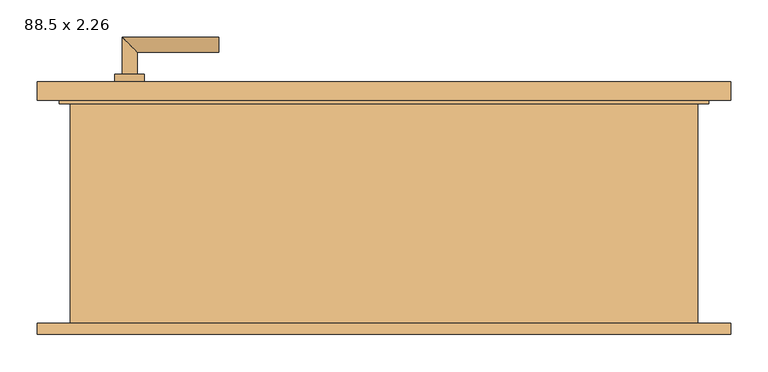
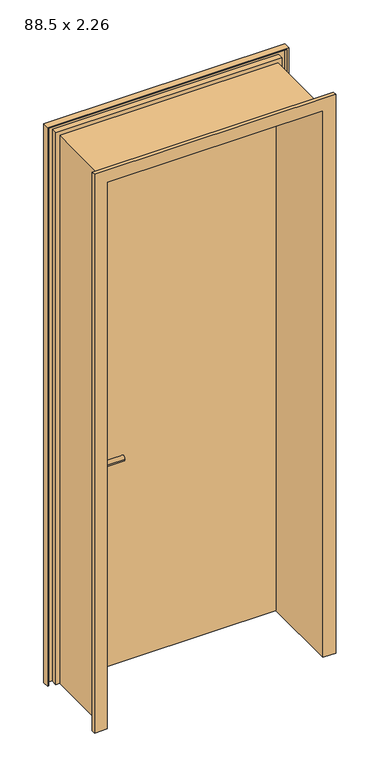
"""IFC4 building model written with IfcOpenShell, lengths in millimetres: door geometry, Drehflügel 1-flg - Stahlzarge : 88.5 x 2.26."""

from ifc_helpers import new_model, si_unit, point, frame, frame_2d, origin, origin_with_axes, place, context, project, spatial, polyline, circle_curve, ellipse_curve, trimmed, segment, composite_curve, outline, extrude, faceted_brep, source, transform, mapped, element, save
from ifc_brep_helpers import plane_surface, cylinder_surface, advanced_brep


def door_88_5_x_2_26_de88e540(model_context):
    return source(origin(), model_context, "Body", "SolidModel", [
        advanced_brep(
        [(-352.5, 139.4346141, 900.0), (-332.5, 139.4346141, 900.0), (-352.5, 69.4346141, 900.0), (-332.5, 89.4346141, 900.0), (-222.5, 69.4346141, 900.0), (-222.5, 89.4346141, 900.0)],
        [
            (0, 1, circle_curve(frame((-342.5, 139.4346141, 900.0), z_axis=(0.0, 1.0, 0.0), x_axis=(1.0, 0.0, 0.0)), 10.0)),
            (1, 0, circle_curve(frame((-342.5, 139.4346141, 900.0), z_axis=(0.0, 1.0, 0.0), x_axis=(1.0, 0.0, 0.0)), 10.0)),
            (0, 2),
            (2, 3, ellipse_curve(frame((-342.5, 79.4346141, 900.0), z_axis=(-0.7071067811865385, 0.7071067811865565, 0.0), x_axis=(0.7071067811865563, 0.7071067811865386, 0.0)), 14.1421356, 10.0)),
            (3, 1),
            (3, 2, ellipse_curve(frame((-342.5, 79.4346141, 900.0), z_axis=(-0.7071067811865385, 0.7071067811865565, 0.0), x_axis=(0.7071067811865563, 0.7071067811865386, 0.0)), 14.1421356, 10.0)),
            (4, 5, circle_curve(frame((-222.5, 79.4346141, 900.0), z_axis=(1.0, 0.0, 0.0), x_axis=(0.0, 1.0, 0.0)), 10.0)),
            (5, 4, circle_curve(frame((-222.5, 79.4346141, 900.0), z_axis=(1.0, 0.0, 0.0), x_axis=(0.0, 1.0, 0.0)), 10.0)),
            (2, 4),
            (5, 3),
        ],
        [
            plane_surface(frame((-342.5, 139.4346141, -387.7526403), z_axis=(0.0, 1.0, 0.0), x_axis=(0.0, 0.0, 1.0))),
            cylinder_surface(frame((-342.5, 139.4346141, 900.0), z_axis=(0.0, 1.0, 0.0), x_axis=(1.0, 0.0, 0.0)), 10.0),
            plane_surface(frame((-222.5, 79.4346141, -387.7526403), z_axis=(1.0, 0.0, 0.0), x_axis=(0.0, 0.0, 1.0))),
            cylinder_surface(frame((-342.5, 79.4346141, 900.0), z_axis=(-1.0, 0.0, 0.0), x_axis=(0.0, 1.0, 0.0)), 10.0),
        ],
        [
            (0, [[1, 2]]),
            (1, [[-1, 3, 4, 5]]),
            (1, [[-2, -5, 6, -3]]),
            (2, [[7, 8]]),
            (3, [[-4, 9, -8, 10]]),
            (3, [[-6, -10, -7, -9]]),
        ],
    ),
        advanced_brep(
        [(-332.5, 199.4346141, 900.0), (-352.5, 199.4346141, 900.0), (-332.5, 229.4346141, 900.0), (-352.5, 249.4346141, 900.0), (-222.5, 229.4346141, 900.0), (-222.5, 249.4346141, 900.0)],
        [
            (0, 1, circle_curve(frame((-342.5, 199.4346141, 900.0), z_axis=(0.0, -1.0, 0.0), x_axis=(-1.0, 0.0, 0.0)), 10.0)),
            (1, 0, circle_curve(frame((-342.5, 199.4346141, 900.0), z_axis=(0.0, -1.0, 0.0), x_axis=(-1.0, 0.0, 0.0)), 10.0)),
            (0, 2),
            (2, 3, ellipse_curve(frame((-342.5, 239.4346141, 900.0), z_axis=(-0.7071067811865475, -0.7071067811865475, 0.0), x_axis=(0.7071067811865474, -0.7071067811865476, 0.0)), 14.1421356, 10.0)),
            (3, 1),
            (3, 2, ellipse_curve(frame((-342.5, 239.4346141, 900.0), z_axis=(-0.7071067811865475, -0.7071067811865475, 0.0), x_axis=(0.7071067811865474, -0.7071067811865476, 0.0)), 14.1421356, 10.0)),
            (4, 5, circle_curve(frame((-222.5, 239.4346141, 900.0), z_axis=(1.0, 0.0, 0.0), x_axis=(0.0, 1.0, 0.0)), 10.0)),
            (5, 4, circle_curve(frame((-222.5, 239.4346141, 900.0), z_axis=(1.0, 0.0, 0.0), x_axis=(0.0, 1.0, 0.0)), 10.0)),
            (2, 4),
            (5, 3),
        ],
        [
            plane_surface(frame((-342.5, 199.4346141, -387.7526403), z_axis=(0.0, -1.0, 0.0), x_axis=(0.0, 0.0, 1.0))),
            cylinder_surface(frame((-342.5, 199.4346141, 900.0), z_axis=(0.0, -1.0, 0.0), x_axis=(-1.0, 0.0, 0.0)), 10.0),
            plane_surface(frame((-222.5, 239.4346141, -387.7526403), z_axis=(1.0, 0.0, 0.0), x_axis=(0.0, 0.0, 1.0))),
            cylinder_surface(frame((-342.5, 239.4346141, 900.0), z_axis=(-1.0, 0.0, 0.0), x_axis=(0.0, 1.0, 0.0)), 10.0),
        ],
        [
            (0, [[1, 2]]),
            (1, [[-1, 3, 4, 5]]),
            (1, [[-2, -5, 6, -3]]),
            (2, [[7, 8]]),
            (3, [[-4, 9, -8, 10]]),
            (3, [[-6, -10, -7, -9]]),
        ],
    ),
        extrude(outline(composite_curve([segment(trimmed(circle_curve(frame_2d((900.0, -342.5)), 20.0), [point((900.0, -362.5))], [point((900.0, -322.5))], False, "CARTESIAN"), True, "CONTINUOUS"), segment(trimmed(circle_curve(frame_2d((900.0, -342.5)), 20.0), [point((900.0, -322.5))], [point((900.0, -362.5))], False, "CARTESIAN"), True, "CONTINUOUS")], self_intersect=False)), frame((0.0, 129.4346141, 0.0), z_axis=(0.0, 1.0, 0.0), x_axis=(0.0, 0.0, 1.0)), (0.0, 0.0, 1.0), 10.0),
        extrude(outline(composite_curve([segment(trimmed(circle_curve(frame_2d((900.0, -342.5)), 20.0), [point((900.0, -362.5))], [point((900.0, -322.5))], False, "CARTESIAN"), True, "CONTINUOUS"), segment(trimmed(circle_curve(frame_2d((900.0, -342.5)), 20.0), [point((900.0, -322.5))], [point((900.0, -362.5))], False, "CARTESIAN"), True, "CONTINUOUS")], self_intersect=False)), frame((0.0, 189.4346141, 0.0), z_axis=(0.0, 1.0, 0.0), x_axis=(0.0, 0.0, 1.0)), (0.0, 0.0, 1.0), 10.0),
        extrude(outline(polyline([(432.5, 164.4346141), (-432.5, 164.4346141), (-432.5, 189.4346141), (432.5, 189.4346141), (432.5, 164.4346141)])), origin_with_axes(), (0.0, 0.0, 1.0), 2250.0),
        faceted_brep([(466.9603207, -150.5653859, 0.0), (417.5, -150.5653859, 0.0), (417.5, 164.4346141, 0.0), (432.5, 164.4346141, 0.0), (432.5, 189.4346141, 0.0), (466.9603207, 189.4346141, 0.0), (466.9603207, 164.4346141, 0.0), (461.9603207, 164.4346141, 0.0), (461.9603207, 184.4346141, 0.0), (437.5, 184.4346141, 0.0), (437.5, 159.4346141, 0.0), (422.5, 159.4346141, 0.0), (422.5, -145.5653859, 0.0), (461.9603207, -145.5653859, 0.0), (461.9603207, -135.5653859, 0.0), (466.9603207, -135.5653859, 0.0), (466.9603207, -150.5653859, 2284.4603207), (-466.9603207, -150.5653859, 2284.4603207), (-466.9603207, -150.5653859, 0.0), (-417.5, -150.5653859, 0.0), (-417.5, -150.5653859, 2235.0), (417.5, -150.5653859, 2235.0), (417.5, 164.4346141, 2235.0), (-417.5, 164.4346141, 2235.0), (-417.5, 164.4346141, 0.0), (-432.5, 164.4346141, 0.0), (-432.5, 164.4346141, 2250.0), (432.5, 164.4346141, 2250.0), (432.5, 189.4346141, 2250.0), (-432.5, 189.4346141, 2250.0), (-432.5, 189.4346141, 0.0), (-466.9603207, 189.4346141, 0.0), (-466.9603207, 189.4346141, 2284.4603207), (466.9603207, 189.4346141, 2284.4603207), (466.9603207, 164.4346141, 2284.4603207), (-466.9603207, 164.4346141, 2284.4603207), (-466.9603207, 164.4346141, 0.0), (-461.9603207, 164.4346141, 0.0), (-461.9603207, 164.4346141, 2279.4603207), (461.9603207, 164.4346141, 2279.4603207), (461.9603207, 184.4346141, 2279.4603207), (-461.9603207, 184.4346141, 2279.4603207), (-461.9603207, 184.4346141, 0.0), (-437.5, 184.4346141, 0.0), (-437.5, 184.4346141, 2255.0), (437.5, 184.4346141, 2255.0), (437.5, 159.4346141, 2255.0), (-437.5, 159.4346141, 2255.0), (-437.5, 159.4346141, 0.0), (-422.5, 159.4346141, 0.0), (-422.5, 159.4346141, 2240.0), (422.5, 159.4346141, 2240.0), (422.5, -145.5653859, 2240.0), (-422.5, -145.5653859, 2240.0), (-422.5, -145.5653859, 0.0), (-461.9603207, -145.5653859, 0.0), (-461.9603207, -145.5653859, 2279.4603207), (461.9603207, -145.5653859, 2279.4603207), (461.9603207, -135.5653859, 2279.4603207), (-461.9603207, -135.5653859, 2279.4603207), (-461.9603207, -135.5653859, 0.0), (-466.9603207, -135.5653859, 0.0), (-466.9603207, -135.5653859, 2284.4603207), (466.9603207, -135.5653859, 2284.4603207)], [[[0, 1, 2, 3, 4, 5, 6, 7, 8, 9, 10, 11, 12, 13, 14, 15]], [[1, 0, 16, 17, 18, 19, 20, 21]], [[2, 1, 21, 22]], [[3, 2, 22, 23, 24, 25, 26, 27]], [[4, 3, 27, 28]], [[5, 4, 28, 29, 30, 31, 32, 33]], [[6, 5, 33, 34]], [[7, 6, 34, 35, 36, 37, 38, 39]], [[8, 7, 39, 40]], [[9, 8, 40, 41, 42, 43, 44, 45]], [[10, 9, 45, 46]], [[11, 10, 46, 47, 48, 49, 50, 51]], [[12, 11, 51, 52]], [[13, 12, 52, 53, 54, 55, 56, 57]], [[14, 13, 57, 58]], [[15, 14, 58, 59, 60, 61, 62, 63]], [[0, 15, 63, 16]], [[17, 62, 61, 18]], [[18, 61, 60, 55, 54, 49, 48, 43, 42, 37, 36, 31, 30, 25, 24, 19]], [[23, 20, 19, 24]], [[29, 26, 25, 30]], [[35, 32, 31, 36]], [[41, 38, 37, 42]], [[47, 44, 43, 48]], [[53, 50, 49, 54]], [[59, 56, 55, 60]], [[22, 21, 20, 23]], [[28, 27, 26, 29]], [[34, 33, 32, 35]], [[40, 39, 38, 41]], [[46, 45, 44, 47]], [[52, 51, 50, 53]], [[58, 57, 56, 59]], [[16, 63, 62, 17]]]),
    ])


if __name__ == "__main__":
    model = new_model("IFC4")
    model_context = context("Model", 3, world=origin())
    ifc_project = project(units=[si_unit("LENGTHUNIT", "METRE", prefix="MILLI")], contexts=[model_context])
    site = spatial("IfcSite", under=ifc_project)
    building = spatial("IfcBuilding", under=site)
    placement = place(None, origin())
    door_88_5_x_2_26_shape = door_88_5_x_2_26_de88e540(model_context)
    element("IfcDoor", 1, ObjectType="Drehflügel 1-flg - Stahlzarge : 88.5 x 2.26", at=placement, inside=building, context=model_context, shape_type="MappedRepresentation", body=[
        mapped(door_88_5_x_2_26_shape, transform((0.0, 0.0, 0.0), x_axis=(1.0, 0.0, 0.0), y_axis=(0.0, 1.0, 0.0), z_axis=(0.0, 0.0, 1.0))),
    ])
    save(model, "model.ifc")

# Revit data of these elements
# Type "Drehflügel 1-flg - Stahlzarge : 88.5 x 2.26"
#   Construction Type Id = "opn-d38"
#   Type Mark = "20"
#   Operation = "SingleSwingRight"
#   Keynote = "16.03"
#   Analytic Construction = "Türfüllung Holz, Sturmtür Metall"
#   Thermal Resistance (R) = 0.270117 (m²·K)/W
#   Heat Transfer Coefficient (U) = 2.3279 W/(m²·K)
#   Rough Width = 0.885 m
#   Rough Height [instance default] = 2.360 m
#   Höhe Türgriff [instance default] = 0.900 m
#   Height = 2.260 m
#   Fußbodenaufbau [instance default] = 0.100 m
#   Width = 0.885 m
#   Sichtbarkeit Sturzlinien [instance default] = yes
#   Türgriff auswählen [instance default] = element 221079
#   Türgriff [instance default] = none
#   Türflügel [instance default] = none
#   Rahmen/Pfosten [instance default] = Metall - Lackiert - Grau
#   Visual Light Transmittance = 0
#   Solar Heat Gain Coefficient = 0
#   Function = (empty or 0)
#   Wall Closure = (empty or 0)
# Element 1 (IfcDoor, "Drehflügel 1-flg - Stahlzarge : 88.5 x 2.26")
#   Rough Height = 2.260 m
#   Fußbodenaufbau = 0.000 m
#   Materials on its faces: "Metall - Lackiert - Grau", "Metall - Chrom", "Holz - Birke"
# Materials
#   "Metall - Lackiert - Grau": class "Farbe 1", colour RGB 98 98 98, transparency 0, Cost = 0
#   "Metall - Chrom": class "Metall", colour RGB 247 247 247, transparency 0, Cost = 0
#   "Holz - Birke": class "Holz", colour RGB 213 164 103, transparency 0, Cost = 0
